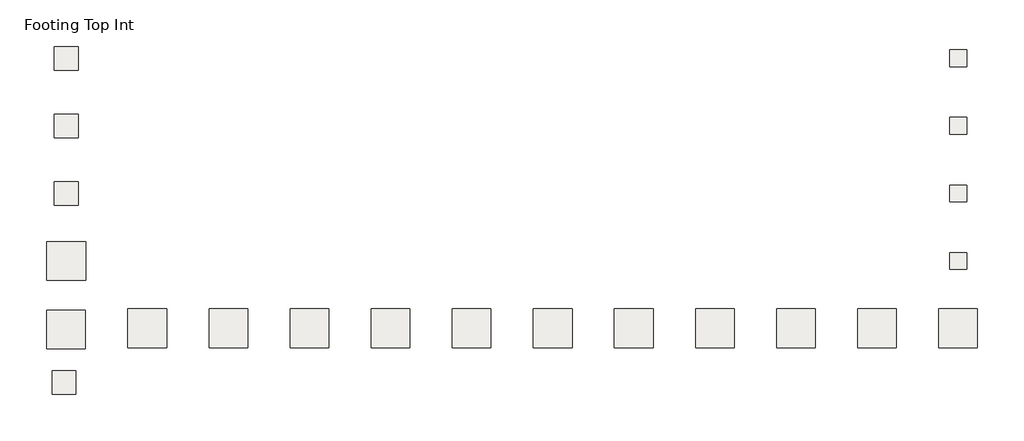
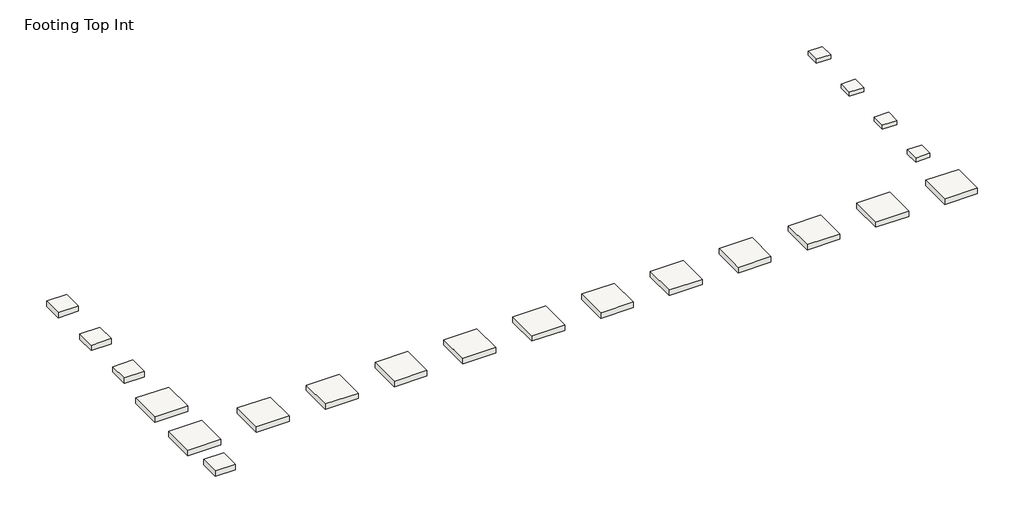
# One storey: 21 slabs.
"""IFC4 building model written with IfcOpenShell, lengths in millimetres."""

from ifc_helpers import new_model, si_unit, frame, origin, place, context, project, spatial, polyline, outline, extrude, faceted_brep, element, save

model = new_model("IFC4")

# Units and contexts
model_context = context("Model", 3, world=origin())
ifc_project = project(units=[si_unit("LENGTHUNIT", "METRE", prefix="MILLI")], contexts=[model_context])

# Site, building, storey
site = spatial("IfcSite", under=ifc_project)
building = spatial("IfcBuilding", under=site)
storey = spatial("IfcBuildingStorey", under=building, Name="Footing Top Int", Elevation=-304.8)

# Slabs
placement = place(None, origin())
element("IfcSlab", 1, ObjectType="Footing-Rectangular : F11", at=placement, inside=storey, context=model_context, shape_type="SweptSolid", body=[
    extrude(outline(polyline([(321470.4398264, -566021.2913841), (324975.6398264, -566021.2913841), (324975.6398264, -569526.4913841), (321470.4398264, -569526.4913841), (321470.4398264, -566021.2913841)])), frame((0.0, 0.0, -914.4), z_axis=(0.0, 0.0, 1.0), x_axis=(1.0, 0.0, 0.0)), (0.0, 0.0, 1.0), 609.6),
])
element("IfcSlab", 2, ObjectType="Footing-Rectangular : F11", at=placement, inside=storey, context=model_context, shape_type="SweptSolid", body=[
    extrude(outline(polyline([(328849.1398264, -565913.3414082), (332354.3398264, -565913.3414082), (332354.3398264, -569418.5414082), (328849.1398264, -569418.5414082), (328849.1398264, -565913.3414082)])), frame((0.0, 0.0, -914.4), z_axis=(0.0, 0.0, 1.0), x_axis=(1.0, 0.0, 0.0)), (0.0, 0.0, 1.0), 609.6),
])
element("IfcSlab", 3, ObjectType="Footing-Rectangular : F11", at=placement, inside=storey, context=model_context, shape_type="SweptSolid", body=[
    extrude(outline(polyline([(336202.4398264, -565913.3414082), (339707.6398264, -565913.3414082), (339707.6398264, -569418.5414082), (336202.4398264, -569418.5414082), (336202.4398264, -565913.3414082)])), frame((0.0, 0.0, -914.4), z_axis=(0.0, 0.0, 1.0), x_axis=(1.0, 0.0, 0.0)), (0.0, 0.0, 1.0), 609.6),
])
element("IfcSlab", 4, ObjectType="Footing-Rectangular : F11", at=placement, inside=storey, context=model_context, shape_type="SweptSolid", body=[
    extrude(outline(polyline([(343555.7398264, -565913.3414082), (347060.9398264, -565913.3414082), (347060.9398264, -569418.5414082), (343555.7398264, -569418.5414082), (343555.7398264, -565913.3414082)])), frame((0.0, 0.0, -914.4), z_axis=(0.0, 0.0, 1.0), x_axis=(1.0, 0.0, 0.0)), (0.0, 0.0, 1.0), 609.6),
])
element("IfcSlab", 5, ObjectType="Footing-Rectangular : F11", at=placement, inside=storey, context=model_context, shape_type="SweptSolid", body=[
    extrude(outline(polyline([(350909.0398264, -565913.3414082), (354414.2398264, -565913.3414082), (354414.2398264, -569418.5414082), (350909.0398264, -569418.5414082), (350909.0398264, -565913.3414082)])), frame((0.0, 0.0, -914.4), z_axis=(0.0, 0.0, 1.0), x_axis=(1.0, 0.0, 0.0)), (0.0, 0.0, 1.0), 609.6),
])
element("IfcSlab", 6, ObjectType="Footing-Rectangular : F11", at=placement, inside=storey, context=model_context, shape_type="SweptSolid", body=[
    extrude(outline(polyline([(358262.3398264, -565913.3414082), (361767.5398264, -565913.3414082), (361767.5398264, -569418.5414082), (358262.3398264, -569418.5414082), (358262.3398264, -565913.3414082)])), frame((0.0, 0.0, -914.4), z_axis=(0.0, 0.0, 1.0), x_axis=(1.0, 0.0, 0.0)), (0.0, 0.0, 1.0), 609.6),
])
element("IfcSlab", 7, ObjectType="Footing-Rectangular : F11", at=placement, inside=storey, context=model_context, shape_type="SweptSolid", body=[
    extrude(outline(polyline([(365615.6398264, -565913.3414082), (369120.8398264, -565913.3414082), (369120.8398264, -569418.5414082), (365615.6398264, -569418.5414082), (365615.6398264, -565913.3414082)])), frame((0.0, 0.0, -914.4), z_axis=(0.0, 0.0, 1.0), x_axis=(1.0, 0.0, 0.0)), (0.0, 0.0, 1.0), 609.6),
])
element("IfcSlab", 8, ObjectType="Footing-Rectangular : F11", at=placement, inside=storey, context=model_context, shape_type="SweptSolid", body=[
    extrude(outline(polyline([(372968.9398264, -565913.3414082), (376474.1398264, -565913.3414082), (376474.1398264, -569418.5414082), (372968.9398264, -569418.5414082), (372968.9398264, -565913.3414082)])), frame((0.0, 0.0, -914.4), z_axis=(0.0, 0.0, 1.0), x_axis=(1.0, 0.0, 0.0)), (0.0, 0.0, 1.0), 609.6),
])
element("IfcSlab", 9, ObjectType="Footing-Rectangular : F11", at=placement, inside=storey, context=model_context, shape_type="SweptSolid", body=[
    extrude(outline(polyline([(380322.2398264, -565913.3414082), (383827.4398264, -565913.3414082), (383827.4398264, -569418.5414082), (380322.2398264, -569418.5414082), (380322.2398264, -565913.3414082)])), frame((0.0, 0.0, -914.4), z_axis=(0.0, 0.0, 1.0), x_axis=(1.0, 0.0, 0.0)), (0.0, 0.0, 1.0), 609.6),
])
element("IfcSlab", 10, ObjectType="Footing-Rectangular : F11", at=placement, inside=storey, context=model_context, shape_type="SweptSolid", body=[
    extrude(outline(polyline([(387675.5398264, -565913.3414082), (391180.7398264, -565913.3414082), (391180.7398264, -569418.5414082), (387675.5398264, -569418.5414082), (387675.5398264, -565913.3414082)])), frame((0.0, 0.0, -914.4), z_axis=(0.0, 0.0, 1.0), x_axis=(1.0, 0.0, 0.0)), (0.0, 0.0, 1.0), 609.6),
])
element("IfcSlab", 11, ObjectType="Footing-Rectangular : F11", at=placement, inside=storey, context=model_context, shape_type="SweptSolid", body=[
    extrude(outline(polyline([(395028.8398264, -565913.3414082), (398534.0398264, -565913.3414082), (398534.0398264, -569418.5414082), (395028.8398264, -569418.5414082), (395028.8398264, -565913.3414082)])), frame((0.0, 0.0, -914.4), z_axis=(0.0, 0.0, 1.0), x_axis=(1.0, 0.0, 0.0)), (0.0, 0.0, 1.0), 609.6),
])
element("IfcSlab", 12, ObjectType="Footing-Rectangular : F11", at=placement, inside=storey, context=model_context, shape_type="SweptSolid", body=[
    extrude(outline(polyline([(402382.1398264, -565913.3414082), (405887.3398264, -565913.3414082), (405887.3398264, -569418.5414082), (402382.1398264, -569418.5414082), (402382.1398264, -565913.3414082)])), frame((0.0, 0.0, -914.4), z_axis=(0.0, 0.0, 1.0), x_axis=(1.0, 0.0, 0.0)), (0.0, 0.0, 1.0), 609.6),
])
element("IfcSlab", 13, ObjectType="Footing-Rectangular : F11", at=placement, inside=storey, context=model_context, shape_type="SweptSolid", body=[
    extrude(outline(polyline([(325010.5648264, -559810.9913841), (325010.5648264, -563316.1913841), (321505.3648264, -563316.1913841), (321505.3648264, -559810.9913841), (325010.5648264, -559810.9913841)])), frame((0.0, 0.0, -914.4), z_axis=(0.0, 0.0, 1.0), x_axis=(1.0, 0.0, 0.0)), (0.0, 0.0, 1.0), 609.6),
])
element("IfcSlab", 14, ObjectType="Footing-Rectangular : F5", at=placement, inside=storey, context=model_context, shape_type="SweptSolid", body=[
    extrude(outline(polyline([(404896.7398264, -542418.3413841), (404896.7398264, -543942.3413841), (403372.7398264, -543942.3413841), (403372.7398264, -542418.3413841), (404896.7398264, -542418.3413841)])), frame((0.0, 0.0, -762.0), z_axis=(0.0, 0.0, 1.0), x_axis=(1.0, 0.0, 0.0)), (0.0, 0.0, 1.0), 457.2),
])
element("IfcSlab", 15, ObjectType="Footing-Rectangular : F5", at=placement, inside=storey, context=model_context, shape_type="SweptSolid", body=[
    extrude(outline(polyline([(404896.7398264, -548546.0913841), (404896.7398264, -550070.0913841), (403372.7398264, -550070.0913841), (403372.7398264, -548546.0913841), (404896.7398264, -548546.0913841)])), frame((0.0, 0.0, -762.0), z_axis=(0.0, 0.0, 1.0), x_axis=(1.0, 0.0, 0.0)), (0.0, 0.0, 1.0), 457.2),
])
element("IfcSlab", 16, ObjectType="Footing-Rectangular : F5", at=placement, inside=storey, context=model_context, shape_type="SweptSolid", body=[
    extrude(outline(polyline([(404896.7398264, -554673.8413841), (404896.7398264, -556197.8413841), (403372.7398264, -556197.8413841), (403372.7398264, -554673.8413841), (404896.7398264, -554673.8413841)])), frame((0.0, 0.0, -762.0), z_axis=(0.0, 0.0, 1.0), x_axis=(1.0, 0.0, 0.0)), (0.0, 0.0, 1.0), 457.2),
])
element("IfcSlab", 17, ObjectType="Footing-Rectangular : F5", at=placement, inside=storey, context=model_context, shape_type="SweptSolid", body=[
    extrude(outline(polyline([(404896.7398264, -560801.5913841), (404896.7398264, -562325.5913841), (403372.7398264, -562325.5913841), (403372.7398264, -560801.5913841), (404896.7398264, -560801.5913841)])), frame((0.0, 0.0, -762.0), z_axis=(0.0, 0.0, 1.0), x_axis=(1.0, 0.0, 0.0)), (0.0, 0.0, 1.0), 457.2),
])
element("IfcSlab", 18, ObjectType="Footing-Rectangular : F7", at=placement, inside=storey, context=model_context, shape_type="Brep", body=[
    faceted_brep([(324121.5648264, -571526.7413841, -304.8), (321987.9648264, -571526.7413841, -304.8), (321987.9648264, -572404.4391729, -304.8), (321987.9648264, -572810.8391729, -304.8), (321987.9648264, -573660.3413841, -304.8), (324121.5648264, -573660.3413841, -304.8), (324121.5648264, -571526.7413841, -914.4), (324121.5648264, -573660.3413841, -914.4), (321987.9648264, -573660.3413841, -914.4), (321987.9648264, -571526.7413841, -914.4)], [[[0, 1, 2, 3, 4, 5]], [[6, 7, 8, 9]], [[1, 0, 6, 9]], [[4, 3, 2, 1, 9, 8]], [[5, 4, 8, 7]], [[0, 5, 7, 6]]]),
])
element("IfcSlab", 19, ObjectType="Footing-Rectangular : F7", at=placement, inside=storey, context=model_context, shape_type="SweptSolid", body=[
    extrude(outline(polyline([(324324.7648264, -542113.5413841), (324324.7648264, -544247.1413841), (322191.1648264, -544247.1413841), (322191.1648264, -542113.5413841), (324324.7648264, -542113.5413841)])), frame((0.0, 0.0, -914.4), z_axis=(0.0, 0.0, 1.0), x_axis=(1.0, 0.0, 0.0)), (0.0, 0.0, 1.0), 609.6),
])
element("IfcSlab", 20, ObjectType="Footing-Rectangular : F7", at=placement, inside=storey, context=model_context, shape_type="SweptSolid", body=[
    extrude(outline(polyline([(324324.7648264, -548241.2913841), (324324.7648264, -550374.8913841), (322191.1648264, -550374.8913841), (322191.1648264, -548241.2913841), (324324.7648264, -548241.2913841)])), frame((0.0, 0.0, -914.4), z_axis=(0.0, 0.0, 1.0), x_axis=(1.0, 0.0, 0.0)), (0.0, 0.0, 1.0), 609.6),
])
element("IfcSlab", 21, ObjectType="Footing-Rectangular : F7", at=placement, inside=storey, context=model_context, shape_type="SweptSolid", body=[
    extrude(outline(polyline([(324324.7648264, -554369.0413841), (324324.7648264, -556502.6413841), (322191.1648264, -556502.6413841), (322191.1648264, -554369.0413841), (324324.7648264, -554369.0413841)])), frame((0.0, 0.0, -914.4), z_axis=(0.0, 0.0, 1.0), x_axis=(1.0, 0.0, 0.0)), (0.0, 0.0, 1.0), 609.6),
])

save(model, "model.ifc")

# Revit data of these elements
# Type "Footing-Rectangular : F11"
#   Assembly Code = "A1010100"
#   Width = 11' - 6"
#   Length = 11' - 6"
#   Thickness = 2' - 0"
#   Structural Material [instance default] = Concrete, Cast-in-Place gray
# Type "Footing-Rectangular : F5"
#   Assembly Code = "A1010100"
#   Width = 5' - 0"
#   Length = 5' - 0"
#   Thickness = 1' - 6"
#   Structural Material [instance default] = Concrete, Cast-in-Place gray
# Type "Footing-Rectangular : F7"
#   Assembly Code = "A1010100"
#   Width = 7' - 0"
#   Length = 7' - 0"
#   Thickness = 2' - 0"
#   Structural Material [instance default] = Concrete, Cast-in-Place gray
# Elements 1, 2, 3, 4, 5, 6, 7, 8, 9, 10, 11, 12, 13 (IfcSlab, "Footing-Rectangular : F11")
#   Comments = ""
#   Structural Material = Concrete, Cast-in-Place gray
#   Phase Created = New Construction
#   Materials on its faces: "Concrete, Cast-in-Place gray"
# Elements 14, 15, 16, 17 (IfcSlab, "Footing-Rectangular : F5")
#   Comments = ""
#   Structural Material = Concrete, Cast-in-Place gray
#   Phase Created = New Construction
#   Materials on its faces: "Concrete, Cast-in-Place gray"
# Elements 18, 19, 20, 21 (IfcSlab, "Footing-Rectangular : F7")
#   Comments = ""
#   Structural Material = Concrete, Cast-in-Place gray
#   Phase Created = New Construction
#   Materials on its faces: "Concrete, Cast-in-Place gray"
# Materials
#   "Concrete, Cast-in-Place gray": class "Concrete", colour RGB 192 192 192, transparency 0, Description = "Cast-in-place concrete", Cost = 0
